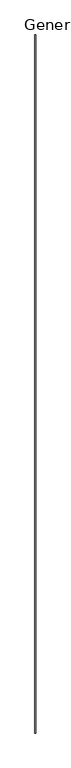
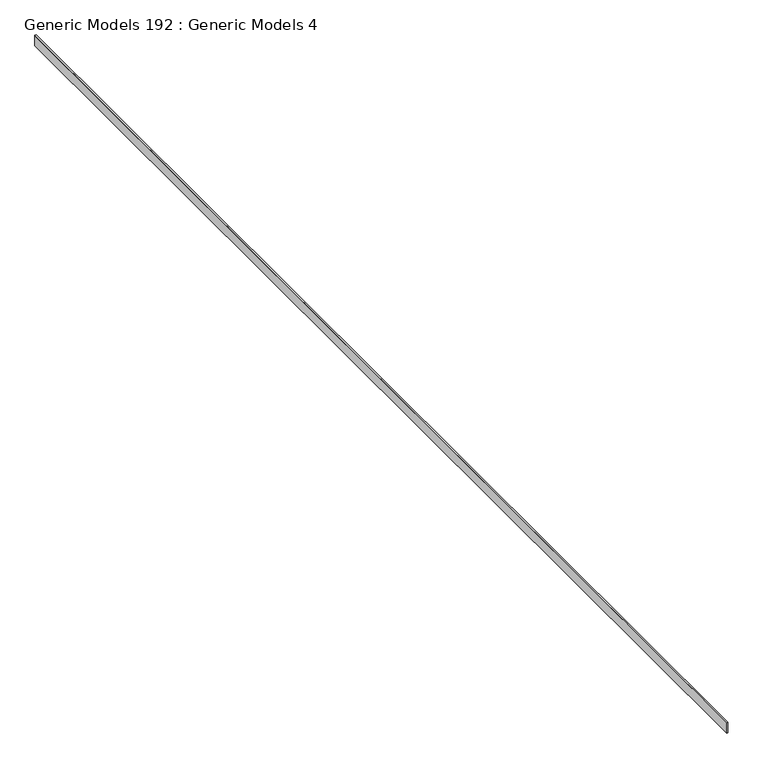
"""IFC4 building model written with IfcOpenShell, lengths in millimetres: proxy geometry, Generic Models 192 : Generic Models 4."""

from ifc_helpers import new_model, si_unit, frame, origin, place, context, project, spatial, polyline, outline, extrude, source, transform, mapped, element, save


def generic_models_192_generic_models_4_5d280612(model_context):
    return source(origin(), model_context, "Body", "SweptSolid", [
        extrude(outline(polyline([(129185.5812308, -5337.5362592), (129357.578074, -5337.5362592), (129357.578074, -5354.5862339), (129354.098274, -5354.5862339), (129354.098274, -5355.8562339), (129185.5812308, -5355.8562339), (129185.5812308, -5337.5362592)])), frame((0.0, -6864.9230338, 0.0), z_axis=(0.0, 1.0, 0.0), x_axis=(0.0, 0.0, 1.0)), (0.0, 0.0, 1.0), 18643.6),
    ])


if __name__ == "__main__":
    model = new_model("IFC4")
    model_context = context("Model", 3, world=origin())
    ifc_project = project(units=[si_unit("LENGTHUNIT", "METRE", prefix="MILLI")], contexts=[model_context])
    site = spatial("IfcSite", under=ifc_project)
    building = spatial("IfcBuilding", under=site)
    placement = place(None, origin())
    generic_models_192_generic_models_4_shape = generic_models_192_generic_models_4_5d280612(model_context)
    element("IfcBuildingElementProxy", 1, Name="Generic Models 192 : Generic Models 4", ObjectType="Generic Models 192 : Generic Models 4", at=placement, inside=building, context=model_context, shape_type="MappedRepresentation", body=[
        mapped(generic_models_192_generic_models_4_shape, transform((0.0, 0.0, 0.0), x_axis=(1.0, 0.0, 0.0), y_axis=(0.0, 1.0, 0.0), z_axis=(0.0, 0.0, 1.0))),
    ])
    save(model, "model.ifc")

# Revit data of these elements
# Element 1 (IfcBuildingElementProxy, "Generic Models 192 : Generic Models 4")
#   Materials on its faces: "_7/8\" SMOOTH TROWEL EXTERIOR STUCCO (COLOR PER OWNER)"
# Materials
#   "_7/8\" SMOOTH TROWEL EXTERIOR STUCCO (COLOR PER OWNER)": class "Generic", colour RGB 233 233 233, transparency 0, Cost = 0
